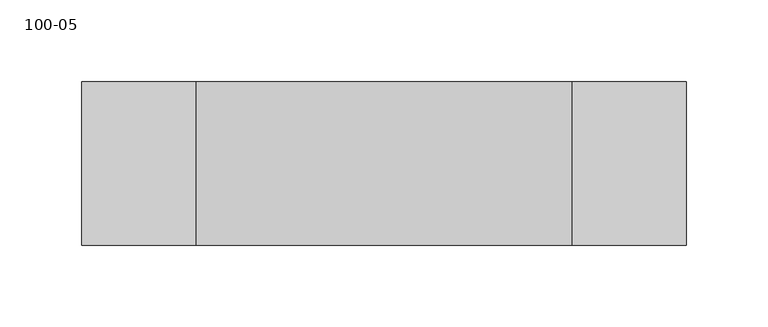
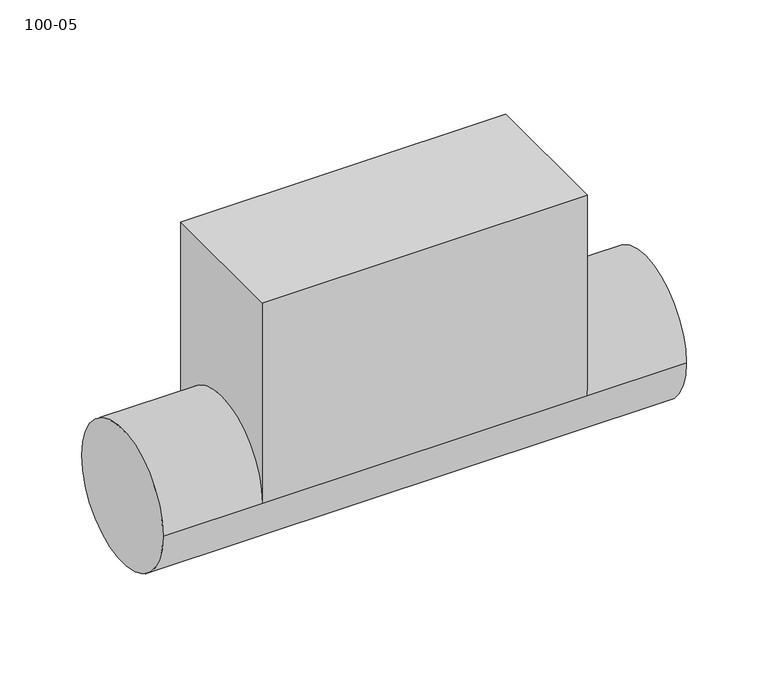
"""IFC4 building model written with IfcOpenShell, lengths in millimetres: proxy geometry, НАГРЕВАТЕЛЬ ЭЛЕКТРИЧЕСКИЙ VKHR-E : 100-05."""

from ifc_helpers import new_model, si_unit, frame, origin, place, context, project, spatial, circle_curve, source, transform, mapped, element, save
from ifc_brep_helpers import plane_surface, cylinder_surface, advanced_brep


def proxy_100_05_01a2785d(model_context):
    return source(origin(), model_context, "Body", "AdvancedBrep", [
        advanced_brep(
        [(370.0, -50.0, 0.0), (370.0, 50.0, 0.0), (0.0, -50.0, 0.0), (0.0, 50.0, 0.0), (300.0, -50.0, 0.0), (70.0, -50.0, 0.0), (70.0, 50.0, 0.0), (300.0, 50.0, 0.0), (300.0, 50.0, 150.0), (70.0, 50.0, 150.0), (70.0, -50.0, 150.0), (300.0, -50.0, 150.0)],
        [
            (0, 1, circle_curve(frame((370.0, 0.0, 0.0), z_axis=(1.0, 0.0, 0.0), x_axis=(0.0, 1.0, 0.0)), 50.0)),
            (1, 0, circle_curve(frame((370.0, 0.0, 0.0), z_axis=(1.0, 0.0, 0.0), x_axis=(0.0, 1.0, 0.0)), 50.0)),
            (2, 3, circle_curve(frame((0.0, 0.0, 0.0), z_axis=(-1.0, 0.0, 0.0), x_axis=(0.0, 1.0, 0.0)), 50.0)),
            (3, 2, circle_curve(frame((0.0, 0.0, 0.0), z_axis=(-1.0, 0.0, 0.0), x_axis=(0.0, 1.0, 0.0)), 50.0)),
            (0, 4),
            (4, 5),
            (5, 2),
            (3, 6),
            (6, 7),
            (7, 1),
            (7, 4, circle_curve(frame((300.0, 0.0, 0.0), z_axis=(1.0, 0.0, 0.0), x_axis=(0.0, 1.0, 0.0)), 50.0)),
            (5, 6, circle_curve(frame((70.0, 0.0, 0.0), z_axis=(-1.0, 0.0, 0.0), x_axis=(0.0, 1.0, 0.0)), 50.0)),
            (8, 9),
            (9, 10),
            (10, 11),
            (11, 8),
            (8, 7),
            (6, 9),
            (5, 10),
            (4, 11),
        ],
        [
            plane_surface(frame((370.0, 50.0, 0.0), z_axis=(1.0, 0.0, 0.0), x_axis=(0.0, 0.0, 1.0))),
            plane_surface(frame((0.0, 50.0, 0.0), z_axis=(-1.0, 0.0, 0.0), x_axis=(0.0, 0.0, -1.0))),
            cylinder_surface(frame((0.0, 0.0, 0.0), z_axis=(1.0, 0.0, 0.0), x_axis=(0.0, 1.0, 0.0)), 50.0),
            plane_surface(frame((70.0, 50.0, 150.0), z_axis=(0.0, 0.0, 1.0), x_axis=(-1.0, 0.0, 0.0))),
            plane_surface(frame((300.0, 50.0, 150.0), z_axis=(0.0, 1.0, 0.0), x_axis=(0.0, 0.0, -1.0))),
            plane_surface(frame((70.0, 50.0, 150.0), z_axis=(-1.0, 0.0, 0.0), x_axis=(0.0, 0.0, -1.0))),
            plane_surface(frame((70.0, -50.0, 150.0), z_axis=(0.0, -1.0, 0.0), x_axis=(0.0, 0.0, -1.0))),
            plane_surface(frame((300.0, -50.0, 150.0), z_axis=(1.0, 0.0, 0.0), x_axis=(0.0, 0.0, -1.0))),
        ],
        [
            (0, [[1, 2]]),
            (1, [[3, 4]]),
            (2, [[-1, 5, 6, 7, -4, 8, 9, 10]]),
            (2, [[-2, -10, 11, -5]]),
            (2, [[-3, -7, 12, -8]]),
            (3, [[13, 14, 15, 16]]),
            (4, [[-13, 17, -9, 18]]),
            (5, [[-14, -18, -12, 19]]),
            (6, [[-15, -19, -6, 20]]),
            (7, [[-16, -20, -11, -17]]),
        ],
    ),
    ])


if __name__ == "__main__":
    model = new_model("IFC4")
    model_context = context("Model", 3, world=origin())
    ifc_project = project(units=[si_unit("LENGTHUNIT", "METRE", prefix="MILLI")], contexts=[model_context])
    site = spatial("IfcSite", under=ifc_project)
    building = spatial("IfcBuilding", under=site)
    placement = place(None, origin())
    proxy_100_05_shape = proxy_100_05_01a2785d(model_context)
    element("IfcBuildingElementProxy", 1, Name="НАГРЕВАТЕЛЬ ЭЛЕКТРИЧЕСКИЙ VKHR-E : 100-05", ObjectType="НАГРЕВАТЕЛЬ ЭЛЕКТРИЧЕСКИЙ VKHR-E : 100-05", at=placement, inside=building, context=model_context, shape_type="MappedRepresentation", body=[
        mapped(proxy_100_05_shape, transform((0.0, 0.0, 0.0), x_axis=(1.0, 0.0, 0.0), y_axis=(0.0, 1.0, 0.0), z_axis=(0.0, 0.0, 1.0))),
    ])
    save(model, "model.ifc")

# Revit data of these elements
# Project information
#   Наименование здания = "Наименование здания"
#   Дата утверждения проекта = "Дата"
#   Заказчик = "Заказчик"
#   Адрес проекта = "Адрес проекта"
#   Наименование проекта = "Наименование проекта"
#   Номер проекта = "Номер проекта"
# Type "НАГРЕВАТЕЛЬ ЭЛЕКТРИЧЕСКИЙ VKHR-E : 100-05"
#   ADSK_Наименование = "Нагреватель электрический VKHR-E"
#   ADSK_Марка = "VKHR-E 100/0,5"
#   L = 370 mm
#   H = 150 mm
#   D = 100 mm
#   Default Elevation = 0
